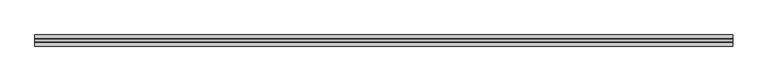
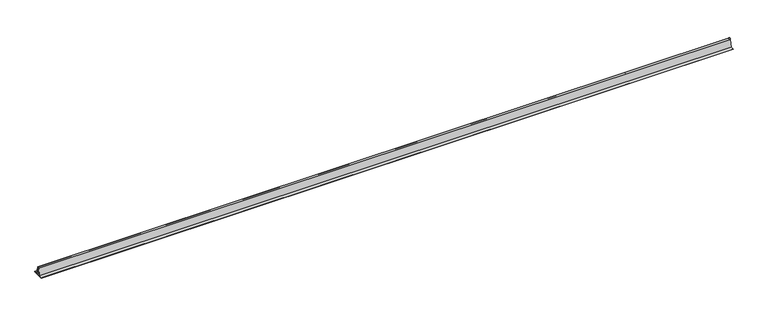
"""IFC4 building model written with IfcOpenShell, lengths in millimetres: proxy geometry, TN_А-профиль, серый : А-профиль h25 (2 м), серый."""

from ifc_helpers import new_model, si_unit, point, frame, frame_2d, origin, place, context, project, spatial, polyline, circle_curve, trimmed, segment, composite_curve, outline, extrude, source, transform, mapped, element, save


def specialty_equipment_d1e2c3e8(model_context):
    return source(origin(), model_context, "Body", "SweptSolid", [
        extrude(outline(composite_curve([segment(polyline([(16.0, 0.0), (-16.0, 0.0), (-16.0, 1.0), (-6.0, 1.0), (-2.9704369, 22.4201248)]), True, "CONTINUOUS"), segment(trimmed(circle_curve(frame_2d((0.0, 22.0)), 3.0), [point((-2.9704369, 22.4201248))], [point((2.9704369, 22.4201248))], False, "CARTESIAN"), True, "CONTINUOUS"), segment(polyline([(2.9704369, 22.4201248), (6.0, 1.0), (16.0, 1.0), (16.0, 0.0)]), True, "CONTINUOUS")], self_intersect=False), holes=[composite_curve([segment(polyline([(-2.9193299, 8.5), (2.9193299, 8.5), (0.9901456, 22.1400416)]), True, "CONTINUOUS"), segment(trimmed(circle_curve(frame_2d((0.0, 22.0)), 1.0), [point((0.9901456, 22.1400416))], [point((-0.9901456, 22.1400416))], True, "CARTESIAN"), True, "CONTINUOUS"), segment(polyline([(-0.9901456, 22.1400416), (-2.9193299, 8.5)]), True, "CONTINUOUS")], self_intersect=False), polyline([(3.1314829, 7.0), (-3.1314829, 7.0), (-3.9800951, 1.0), (3.9800951, 1.0), (3.1314829, 7.0)])]), frame((0.0, 0.0, 0.0), z_axis=(1.0, 0.0, 0.0), x_axis=(0.0, 1.0, 0.0)), (0.0, 0.0, 1.0), 2000.0),
    ])


if __name__ == "__main__":
    model = new_model("IFC4")
    model_context = context("Model", 3, world=origin())
    ifc_project = project(units=[si_unit("LENGTHUNIT", "METRE", prefix="MILLI")], contexts=[model_context])
    site = spatial("IfcSite", under=ifc_project)
    building = spatial("IfcBuilding", under=site)
    placement = place(None, origin())
    specialty_equipment_shape = specialty_equipment_d1e2c3e8(model_context)
    element("IfcBuildingElementProxy", 1, Name="TN_А-профиль, серый : А-профиль h25 (2 м), серый", ObjectType="TN_А-профиль, серый : А-профиль h25 (2 м), серый", at=placement, inside=building, context=model_context, shape_type="MappedRepresentation", body=[
        mapped(specialty_equipment_shape, transform((0.0, 0.0, 0.0), x_axis=(1.0, 0.0, 0.0), y_axis=(0.0, 1.0, 0.0), z_axis=(0.0, 0.0, 1.0))),
    ])
    save(model, "model.ifc")

# Revit data of these elements
# Type "TN_А-профиль, серый : А-профиль h25 (2 м), серый"
#   Description = "А-профиль из ПВХ. СТО 72746455-3.9.5-2017. А-профиль применяется на кровлях из ПВХ мембран для имитации внешнего вида фальцевой кровли. Это позволяет получить не шумящую во время дождя и более надёжную кровлю, идентичную по внешнему виду металлической кровле. рименяется совместно с ПВХ мембранами LOGICROOF и ECOPLAST. Приваривается к мембране гомогенно при помощи горячего воздуха. Длина профиля 2 м, упаковывается в картонные коробки, 50 шт. в коробке."
#   Type Comments = "п.м."
#   Manufacturer = "ТехноНИКОЛЬ"
#   URL = "https://nav.tn.ru/catalog/krovlya/komplektatsiya-dlya-krovli/a-profil-iz-pvkh/?sphrase_id=266377"
#   ADSK_Примечание = ""
#   ADSK_Обозначение [instance default] = "ТехноНИКОЛЬ"
#   ADSK_Наименование = "А-профиль (2 м), серый"
#   ADSK_Масса_Текст = ""
#   ADSK_Марка = ""
#   ADSK_Код изделия = "551279"
#   ADSK_Завод-изготовитель [instance default] = "ТехноНИКОЛЬ"
#   ADSK_Единица измерения [instance default] = "п.м."
#   ADSK_Группирование = "Комплектующие и воронки"
#   ADSK_URL страницы изделия = "https://nav.tn.ru/catalog/krovlya/komplektatsiya-dlya-krovli/a-profil-iz-pvkh/?sphrase_id=266377"
#   ADSK_URL документации изделия = "https://nav.tn.ru/upload/iblock/7bd/Tekhlist-7.58_A_profil_rus.pdf"
#   built-in parameter 1001306 [instance default] = 3.28084 (stored number, unit not read)
#   ADSK_Размер_Длина [instance default] = 1000 mm
#   ADSK_Количество [instance default] = 1
#   Видимость_Тип профиля 50 = no
#   Видимость_Тип профиля 25 = yes
#   Материал = TN_ПВХ_Серый
#   Default Elevation = 0
# Element 1 (IfcBuildingElementProxy, "TN_А-профиль, серый : А-профиль h25 (2 м), серый")
#   built-in parameter 1001306 = 6.56168 (stored number, unit not read)
#   ADSK_Размер_Длина = 2000 mm
#   ADSK_Количество = 2
#   Materials on its faces: "TN_ПВХ_Серый"
# Materials
#   "TN_ПВХ_Серый": class "Типовые", colour RGB 192 192 192, transparency 0, Cost = 0
